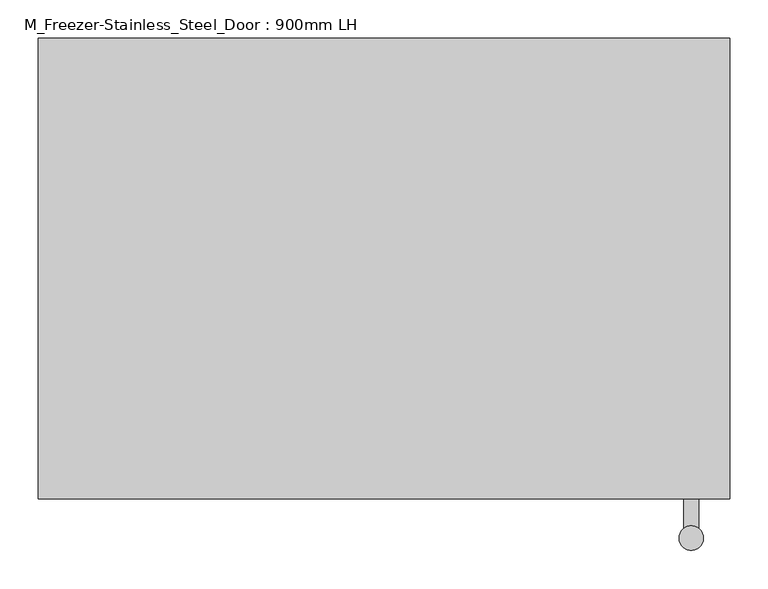
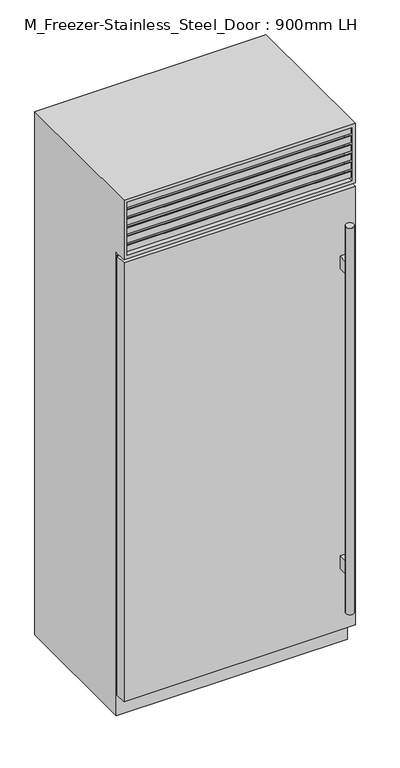
"""IFC4 building model written with IfcOpenShell, lengths in millimetres: proxy geometry, M_Freezer-Stainless_Steel_Door : 900mm LH."""

from ifc_helpers import new_model, si_unit, frame, origin, place, context, project, spatial, polyline, circle_curve, ellipse_curve, outline, extrude, faceted_brep, source, transform, mapped, element, save
from ifc_brep_helpers import plane_surface, cylinder_surface, advanced_brep


def m_freezer_stainless_steel_door_900mm_lh_c3cb7a96(model_context):
    return source(origin(), model_context, "Body", "SolidModel", [
        extrude(outline(polyline([(-450.0, -655.55), (450.0, -655.55), (450.0, -700.0), (-450.0, -700.0), (-450.0, -655.55)])), frame((0.0, 0.0, 88.9), z_axis=(0.0, 0.0, 1.0), x_axis=(1.0, 0.0, 0.0)), (0.0, 0.0, 1.0), 1803.925),
        faceted_brep([(450.0, -700.0, 2150.0), (-450.0, -700.0, 2150.0), (-450.0, -700.0, 1905.525), (450.0, -700.0, 1905.525), (437.3, -700.0, 2137.3), (437.3, -700.0, 1918.225), (-437.3, -700.0, 1918.225), (-437.3, -700.0, 2137.3), (450.0, -100.0, 2150.0), (-450.0, -100.0, 2150.0), (-450.0, -100.0, 0.0), (-450.0, -649.2, 0.0), (-450.0, -649.2, 1905.525), (450.0, -649.2, 1905.525), (450.0, -649.2, 0.0), (450.0, -100.0, 0.0), (-437.3, -649.2, 2137.3), (437.3, -649.2, 2137.3), (-437.3, -649.2, 1918.225), (437.3, -649.2, 1918.225)], [[[0, 1, 2, 3], [4, 5, 6, 7]], [[1, 0, 8, 9]], [[2, 1, 9, 10, 11, 12]], [[3, 2, 12, 13]], [[8, 0, 3, 13, 14, 15]], [[4, 7, 16, 17]], [[7, 6, 18, 16]], [[6, 5, 19, 18]], [[5, 4, 17, 19]], [[15, 14, 11, 10]], [[9, 8, 15, 10]], [[17, 16, 18, 19]], [[11, 14, 13, 12]]]),
        extrude(outline(polyline([(-649.2, 1918.225), (-696.825, 1930.9860803), (-696.825, 1956.3860803), (-693.65, 1956.3860803), (-693.65, 1933.5368938), (-649.2, 1921.6265522), (-649.2, 1918.225)])), frame((-437.3, 0.0, 0.0), z_axis=(1.0, 0.0, 0.0), x_axis=(0.0, 1.0, 0.0)), (0.0, 0.0, 1.0), 874.6),
        extrude(outline(polyline([(-649.2, 1954.4077839), (-696.825, 1967.1688642), (-696.825, 1992.5688642), (-693.65, 1992.5688642), (-693.65, 1969.7196777), (-649.2, 1957.8093361), (-649.2, 1954.4077839)])), frame((-437.3, 0.0, 0.0), z_axis=(1.0, 0.0, 0.0), x_axis=(0.0, 1.0, 0.0)), (0.0, 0.0, 1.0), 874.6),
        extrude(outline(polyline([(-649.2, 1990.5905679), (-696.825, 2003.3516482), (-696.825, 2028.7516482), (-693.65, 2028.7516482), (-693.65, 2005.9024616), (-649.2, 1993.99212), (-649.2, 1990.5905679)])), frame((-437.3, 0.0, 0.0), z_axis=(1.0, 0.0, 0.0), x_axis=(0.0, 1.0, 0.0)), (0.0, 0.0, 1.0), 874.6),
        extrude(outline(polyline([(-649.2, 2026.7733518), (-696.825, 2039.5344321), (-696.825, 2064.9344321), (-693.65, 2064.9344321), (-693.65, 2042.0852456), (-649.2, 2030.174904), (-649.2, 2026.7733518)])), frame((-437.3, 0.0, 0.0), z_axis=(1.0, 0.0, 0.0), x_axis=(0.0, 1.0, 0.0)), (0.0, 0.0, 1.0), 874.6),
        extrude(outline(polyline([(-649.2, 2062.9561358), (-696.825, 2075.7172161), (-696.825, 2101.1172161), (-693.65, 2101.1172161), (-693.65, 2078.2680295), (-649.2, 2066.3576879), (-649.2, 2062.9561358)])), frame((-437.3, 0.0, 0.0), z_axis=(1.0, 0.0, 0.0), x_axis=(0.0, 1.0, 0.0)), (0.0, 0.0, 1.0), 874.6),
        extrude(outline(polyline([(-649.2, 2099.1389197), (-696.825, 2111.9), (-696.825, 2137.3), (-693.65, 2137.3), (-693.65, 2114.4508135), (-649.2, 2102.5404719), (-649.2, 2099.1389197)])), frame((-437.3, 0.0, 0.0), z_axis=(1.0, 0.0, 0.0), x_axis=(0.0, 1.0, 0.0)), (0.0, 0.0, 1.0), 874.6),
        advanced_brep(
        [(-446.825, -655.55, 1889.65), (-446.825, -649.2, 1889.65), (-446.825, -649.2, 92.075), (-446.825, -655.55, 92.075), (-443.65, -649.2, 1886.475), (-443.65, -655.55, 1886.475), (-443.65, -655.55, 95.25), (-443.65, -649.2, 95.25), (446.825, -649.2, 92.075), (446.825, -655.55, 92.075), (443.65, -655.55, 95.25), (443.65, -649.2, 95.25), (446.825, -649.2, 1889.65), (446.825, -655.55, 1889.65), (443.65, -655.55, 1886.475), (443.65, -649.2, 1886.475)],
        [
            (0, 1, ellipse_curve(frame((-446.825, -652.375, 1889.65), z_axis=(-0.7071067811865476, 0.0, -0.7071067811865475), x_axis=(-0.7071067811865474, 0.0, 0.7071067811865476)), 4.4901281, 3.175)),
            (1, 2),
            (2, 3, ellipse_curve(frame((-446.825, -652.375, 92.075), z_axis=(-0.7071067811865475, 0.0, 0.7071067811865476), x_axis=(0.7071067811865476, 0.0, 0.7071067811865474)), 4.4901281, 3.175)),
            (3, 0),
            (4, 5),
            (5, 6),
            (6, 7),
            (7, 4),
            (2, 8),
            (8, 9, ellipse_curve(frame((446.825, -652.375, 92.075), z_axis=(-0.7071067811865476, 0.0, -0.7071067811865475), x_axis=(-0.7071067811865474, 0.0, 0.7071067811865476)), 4.4901281, 3.175)),
            (9, 3),
            (6, 10),
            (10, 11),
            (11, 7),
            (8, 12),
            (12, 13, ellipse_curve(frame((446.825, -652.375, 1889.65), z_axis=(0.7071067811865474, 0.0, -0.7071067811865476), x_axis=(-0.7071067811865475, 0.0, -0.7071067811865475)), 4.4901281, 3.175)),
            (13, 9),
            (10, 14),
            (14, 15),
            (15, 11),
            (1, 12),
            (15, 4),
            (0, 13),
            (5, 14),
        ],
        [
            cylinder_surface(frame((-446.825, -652.375, 1892.825), z_axis=(0.0, 0.0, 1.0), x_axis=(0.0, -1.0, 0.0)), 3.175),
            plane_surface(frame((-443.65, -655.55, 1886.475), z_axis=(1.0, 0.0, 0.0), x_axis=(0.0, 0.0, -1.0))),
            cylinder_surface(frame((-450.0, -652.375, 92.075), z_axis=(-1.0, 0.0, 0.0), x_axis=(0.0, -1.0, 0.0)), 3.175),
            plane_surface(frame((-443.65, -655.55, 95.25), z_axis=(0.0, 0.0, 1.0), x_axis=(1.0, 0.0, 0.0))),
            cylinder_surface(frame((446.825, -652.375, 88.9), z_axis=(0.0, 0.0, -1.0), x_axis=(0.0, -1.0, 0.0)), 3.175),
            plane_surface(frame((443.65, -655.55, 95.25), z_axis=(-1.0, 0.0, 0.0), x_axis=(0.0, 0.0, 1.0))),
            plane_surface(frame((443.65, -649.2, 1886.475), z_axis=(0.0, 1.0, 0.0), x_axis=(-1.0, 0.0, 0.0))),
            cylinder_surface(frame((450.0, -652.375, 1889.65), z_axis=(1.0, 0.0, 0.0), x_axis=(0.0, -1.0, 0.0)), 3.175),
            plane_surface(frame((446.825, -655.55, 1889.65), z_axis=(0.0, -1.0, 0.0), x_axis=(-1.0, 0.0, 0.0))),
            plane_surface(frame((443.65, -655.55, 1886.475), z_axis=(0.0, 0.0, -1.0), x_axis=(-1.0, 0.0, 0.0))),
        ],
        [
            (0, [[1, 2, 3, 4]]),
            (1, [[5, 6, 7, 8]]),
            (2, [[-3, 9, 10, 11]]),
            (3, [[-7, 12, 13, 14]]),
            (4, [[-10, 15, 16, 17]]),
            (5, [[-13, 18, 19, 20]]),
            (6, [[21, -15, -9, -2], [-14, -20, 22, -8]]),
            (7, [[-16, -21, -1, 23]]),
            (8, [[-11, -17, -23, -4], [24, -18, -12, -6]]),
            (9, [[-19, -24, -5, -22]]),
        ],
    ),
        advanced_brep(
        [(409.525, -700.0, 1626.125), (409.525, -700.0, 1575.325), (390.475, -700.0, 1575.325), (390.475, -700.0, 1626.125), (409.525, -700.0, 393.7), (409.525, -700.0, 342.9), (390.475, -700.0, 342.9), (390.475, -700.0, 393.7), (409.525, -738.4741958, 1626.125), (409.525, -738.4741958, 1575.325), (390.475, -738.4741958, 1575.325), (390.475, -738.4741958, 1626.125), (409.525, -738.4741958, 393.7), (409.525, -738.4741958, 342.9), (390.475, -738.4741958, 342.9), (390.475, -738.4741958, 393.7), (384.125, -751.1741958, 1778.525), (415.875, -751.1741958, 1778.525), (384.125, -751.1741958, 190.5), (415.875, -751.1741958, 190.5)],
        [
            (0, 1),
            (1, 2),
            (2, 3),
            (3, 0),
            (4, 5),
            (5, 6),
            (6, 7),
            (7, 4),
            (0, 8),
            (8, 9),
            (9, 1),
            (9, 10, circle_curve(frame((400.0, -751.1741958, 1575.325), z_axis=(0.0, 0.0, 1.0), x_axis=(1.0, 0.0, 0.0)), 15.875)),
            (10, 2),
            (10, 11),
            (11, 3),
            (11, 8, circle_curve(frame((400.0, -751.1741958, 1626.125), z_axis=(0.0, 0.0, -1.0), x_axis=(1.0, 0.0, 0.0)), 15.875)),
            (4, 12),
            (12, 13),
            (13, 5),
            (13, 14, circle_curve(frame((400.0, -751.1741958, 342.9), z_axis=(0.0, 0.0, 1.0), x_axis=(1.0, 0.0, 0.0)), 15.875)),
            (14, 6),
            (14, 15),
            (15, 7),
            (15, 12, circle_curve(frame((400.0, -751.1741958, 393.7), z_axis=(0.0, 0.0, -1.0), x_axis=(1.0, 0.0, 0.0)), 15.875)),
            (16, 17, circle_curve(frame((400.0, -751.1741958, 1778.525), z_axis=(0.0, 0.0, 1.0), x_axis=(1.0, 0.0, 0.0)), 15.875)),
            (17, 16, circle_curve(frame((400.0, -751.1741958, 1778.525), z_axis=(0.0, 0.0, 1.0), x_axis=(1.0, 0.0, 0.0)), 15.875)),
            (18, 19, circle_curve(frame((400.0, -751.1741958, 190.5), z_axis=(0.0, 0.0, -1.0), x_axis=(1.0, 0.0, 0.0)), 15.875)),
            (19, 18, circle_curve(frame((400.0, -751.1741958, 190.5), z_axis=(0.0, 0.0, -1.0), x_axis=(1.0, 0.0, 0.0)), 15.875)),
            (16, 18),
            (19, 17),
        ],
        [
            plane_surface(frame((409.525, -700.0, 1626.125), z_axis=(0.0, 1.0, 0.0), x_axis=(0.0, 0.0, -1.0))),
            plane_surface(frame((409.525, -700.0, 1626.125), z_axis=(1.0, 0.0, 0.0), x_axis=(0.0, -1.0, 0.0))),
            plane_surface(frame((409.525, -700.0, 1575.325), z_axis=(0.0, 0.0, -1.0), x_axis=(0.0, -1.0, 0.0))),
            plane_surface(frame((390.475, -700.0, 1575.325), z_axis=(-1.0, 0.0, 0.0), x_axis=(0.0, -1.0, 0.0))),
            plane_surface(frame((390.475, -700.0, 1626.125), z_axis=(0.0, 0.0, 1.0), x_axis=(0.0, -1.0, 0.0))),
            plane_surface(frame((409.525, -700.0, 393.7), z_axis=(1.0, 0.0, 0.0), x_axis=(0.0, -1.0, 0.0))),
            plane_surface(frame((409.525, -700.0, 342.9), z_axis=(0.0, 0.0, -1.0), x_axis=(0.0, -1.0, 0.0))),
            plane_surface(frame((390.475, -700.0, 342.9), z_axis=(-1.0, 0.0, 0.0), x_axis=(0.0, -1.0, 0.0))),
            plane_surface(frame((390.475, -700.0, 393.7), z_axis=(0.0, 0.0, 1.0), x_axis=(0.0, -1.0, 0.0))),
            plane_surface(frame((415.875, -751.1741958, 1778.525), z_axis=(0.0, 0.0, 1.0), x_axis=(0.0, 1.0, 0.0))),
            plane_surface(frame((415.875, -751.1741958, 190.5), z_axis=(0.0, 0.0, -1.0), x_axis=(0.0, -1.0, 0.0))),
            cylinder_surface(frame((400.0, -751.1741958, 190.5), z_axis=(0.0, 0.0, 1.0), x_axis=(1.0, 0.0, 0.0)), 15.875),
        ],
        [
            (0, [[1, 2, 3, 4]]),
            (0, [[5, 6, 7, 8]]),
            (1, [[-1, 9, 10, 11]]),
            (2, [[-2, -11, 12, 13]]),
            (3, [[-3, -13, 14, 15]]),
            (4, [[-4, -15, 16, -9]]),
            (5, [[-5, 17, 18, 19]]),
            (6, [[-6, -19, 20, 21]]),
            (7, [[-7, -21, 22, 23]]),
            (8, [[-8, -23, 24, -17]]),
            (9, [[25, 26]]),
            (10, [[27, 28]]),
            (11, [[-25, 29, -28, 30]]),
            (11, [[-26, -30, -27, -29], [-10, -16, -14, -12], [-18, -24, -22, -20]]),
        ],
    ),
    ])


if __name__ == "__main__":
    model = new_model("IFC4")
    model_context = context("Model", 3, world=origin())
    ifc_project = project(units=[si_unit("LENGTHUNIT", "METRE", prefix="MILLI")], contexts=[model_context])
    site = spatial("IfcSite", under=ifc_project)
    building = spatial("IfcBuilding", under=site)
    placement = place(None, origin())
    m_freezer_stainless_steel_door_900mm_lh_shape = m_freezer_stainless_steel_door_900mm_lh_c3cb7a96(model_context)
    element("IfcBuildingElementProxy", 1, Name="M_Freezer-Stainless_Steel_Door : 900mm LH", ObjectType="M_Freezer-Stainless_Steel_Door : 900mm LH", at=placement, inside=building, context=model_context, shape_type="MappedRepresentation", body=[
        mapped(m_freezer_stainless_steel_door_900mm_lh_shape, transform((0.0, 0.0, 0.0), x_axis=(1.0, 0.0, 0.0), y_axis=(0.0, 1.0, 0.0), z_axis=(0.0, 0.0, 1.0))),
    ])
    save(model, "model.ifc")

# Revit data of these elements
# Type "M_Freezer-Stainless_Steel_Door : 900mm LH"
#   Label = "Freezer"
#   Description = "Stainless Steel Door Freezer"
#   Assembly Code = "E1090320"
#   Width = 0.9 m
#   Wall Offset = 0.1 m
#   Voltage = 120 V
#   Power Consumption = 1000 VA
#   Height = 2.15 m
#   Handle Centerline = 0.85 m
#   Depth = 0.6 m
#   Amperage = 8.33333 A
#   Show Label = yes
#   RH = no
#   LH = yes
#   Gasket = Appliance - Gasket
#   Appliance Finish = Appliance - Stainless Steel
#   Type Comments = ""
#   Default Elevation = 0
# Element 1 (IfcBuildingElementProxy, "M_Freezer-Stainless_Steel_Door : 900mm LH")
#   Materials on its faces: "Appliance - Stainless Steel", "Appliance - Gasket"
# Materials
#   "Appliance - Gasket": class "Miscellaneous", colour RGB 234 234 234, transparency 0, Cost = 0
#   "Appliance - Stainless Steel": class "Metal", colour RGB 189 187 185, transparency 0, Description = "Stainless Steel 18/8", Cost = 0
